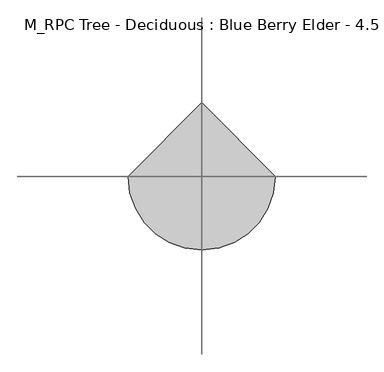
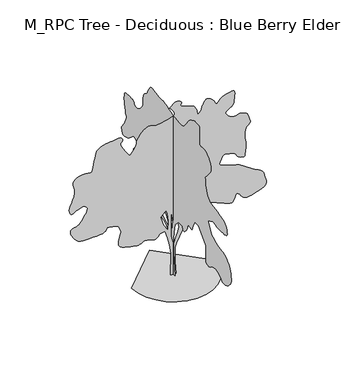
"""IFC4 building model written with IfcOpenShell, lengths in millimetres: geographic element geometry, M_RPC Tree - Deciduous : Blue Berry Elder - 4.5 Meters."""

from ifc_helpers import new_model, si_unit, origin, place, context, project, spatial, triangles, source, transform, mapped, element, save


def m_rpc_tree_deciduous_blue_berry_elder_4_5_meters_08da9c25(model_context):
    return source(origin(), model_context, "Body", "Tessellation", [
        triangles([(-0.0014684, 58.7037978, 0.0041346), (-0.0014684, -62.498052, 0.0041346), (-0.0014684, -15.3641626, 565.6129683), (-0.0014684, -1.8971866, 909.0182064), (-0.0014684, -22.0974929, 1104.2884094), (-0.0014684, -75.9650625, 1326.4911255), (-0.0014684, -224.1009287, 1474.6287403), (-0.0014684, -378.970291, 1474.6287403), (-0.0014684, -412.6378218, 1380.3586224), (-0.0014684, -479.9703761, 1387.0936764), (-0.0014684, -554.0404552, 1474.6287403), (-0.0014684, -601.1729708, 1568.8962421), (-0.0014684, -628.1080273, 1663.1638893), (-0.0014684, -702.1755266, 1636.2313763), (-0.0014684, -782.9756092, 1629.4963223), (-0.0014684, -857.0431812, 1797.8338669), (-0.0014684, -910.9107508, 1898.833952), (-0.0014684, -1059.0483656, 1892.1015141), (-0.0014684, -1173.5159426, 1797.8338669), (-0.0014684, -1382.2535648, 1575.6288254), (-0.0014684, -1388.9861481, 1353.4261093), (-0.0014684, -1386.9236286, 1327.021035), (-0.0014684, -1382.3910564, 1295.553479), (-0.0014684, -1377.8561588, 1261.3760593), (-0.0014684, -1375.7936394, 1226.8434288), (-0.0014684, -1378.6786377, 1194.3159811), (-0.0014684, -1388.9861481, 1166.1458982), (-0.0014684, -1409.1860779, 1144.6884144), (-0.0014684, -1434.4711624, 1129.1809307), (-0.0014684, -1458.931152, 1117.9109064), (-0.0014684, -1483.3911415, 1111.8258854), (-0.0014684, -1508.676226, 1111.8658539), (-0.0014684, -1535.6112099, 1118.9734142), (-0.0014684, -1565.0162464, 1134.0884073), (-0.0014684, -1597.723843, 1158.1559063), (-0.0014684, -1638.2812511, 1183.6959171), (-0.0014684, -1688.0263252, 1202.5209309), (-0.0014684, -1742.9539318, 1214.5159836), (-0.0014684, -1799.0589375, 1219.5610245), (-0.0014684, -1852.3364994, 1217.5409443), (-0.0014684, -1898.783955, 1208.3334394), (-0.0014684, -1934.3939907, 1191.8234734), (-0.0014684, -1963.8416119, 1167.0484594), (-0.0014684, -1995.1715309, 1136.2684341), (-0.0014684, -2029.446619, 1104.1908863), (-0.0014684, -2067.729166, 1075.5283916), (-0.0014684, -2111.0741947, 1054.9958513), (-0.0014684, -2160.5442856, 1047.2983561), (-0.0014684, -2217.1992577, 1057.1533504), (-0.0014684, -2275.1493542, 1083.4008762), (-0.0014684, -2327.094294, 1119.5408941), (-0.0014684, -2371.9694618, 1162.2784018), (-0.0014684, -2408.7193989, 1208.3134552), (-0.0014684, -2436.2819607, 1254.348436), (-0.0014684, -2453.5944214, 1297.0834728), (-0.0014684, -2459.6019035, 1333.2260342), (-0.0014684, -2455.754464, 1372.7236233), (-0.0014684, -2445.3120781, 1424.1161259), (-0.0014684, -2429.919413, 1481.9887562), (-0.0014684, -2411.2318909, 1540.9212055), (-0.0014684, -2390.8944695, 1595.4962173), (-0.0014684, -2370.5569027, 1640.2937737), (-0.0014684, -2351.8669098, 1669.8963272), (-0.0014684, -2330.1568977, 1694.4363991), (-0.0014684, -2300.1992786, 1725.2163517), (-0.0014684, -2262.8217636, 1758.5913494), (-0.0014684, -2218.8493023, 1790.903912), (-0.0014684, -2169.1042282, 1818.5039715), (-0.0014684, -2114.4116364, 1837.74146), (-0.0014684, -2055.5966217, 1844.9664551), (-0.0014684, -1994.4066067, 1849.8740044), (-0.0014684, -1932.1564819, 1863.6164795), (-0.0014684, -1869.0239983, 1884.7189705), (-0.0014684, -1805.1839996, 1911.7115089), (-0.0014684, -1740.8139462, 1943.1215103), (-0.0014684, -1676.0888271, 1977.4765354), (-0.0014684, -1611.1887188, 2013.3016743), (-0.0014684, -1469.786158, 2275.9068661), (-0.0014684, -1685.2562908, 2376.9094219), (-0.0014684, -1714.2713802, 2368.3093655), (-0.0014684, -1744.228854, 2360.0643745), (-0.0014684, -1776.0713871, 2352.5268986), (-0.0014684, -1810.7388931, 2346.049387), (-0.0014684, -1849.1765179, 2340.9844345), (-0.0014684, -1892.3265003, 2337.686816), (-0.0014684, -1941.1290447, 2336.5068008), (-0.0014684, -1996.881601, 2336.291843), (-0.0014684, -2057.3441895, 2336.4293346), (-0.0014684, -2118.1616982, 2338.0968201), (-0.0014684, -2174.9742188, 2342.4769306), (-0.0014684, -2223.421843, 2350.7393623), (-0.0014684, -2259.1517841, 2364.0693626), (-0.0014684, -2277.7993378, 2383.6418598), (-0.0014684, -2281.3742649, 2414.4819832), (-0.0014684, -2275.8767807, 2457.2194908), (-0.0014684, -2262.9592552, 2506.4269524), (-0.0014684, -2244.2692623, 2556.7020813), (-0.0014684, -2221.4593174, 2602.6271851), (-0.0014684, -2196.1742329, 2638.7770134), (-0.0014684, -2170.0641987, 2659.7021896), (-0.0014684, -2143.7191498, 2670.2021301), (-0.0014684, -2115.1367374, 2679.2771576), (-0.0014684, -2082.0791622, 2687.9772079), (-0.0014684, -2042.3065899, 2697.4022141), (-0.0014684, -1993.581657, 2708.6021118), (-0.0014684, -1933.6665642, 2722.6021294), (-0.0014684, -1860.3264187, 2740.5021996), (-0.0014684, -1781.7239491, 2758.3022758), (-0.0014684, -1708.0688519, 2773.1522415), (-0.0014684, -1640.1837513, 2787.8522163), (-0.0014684, -1578.8962132, 2805.302314), (-0.0014684, -1525.0287163, 2828.2773651), (-0.0014684, -1479.4062103, 2859.6021973), (-0.0014684, -1442.8536449, 2902.1272179), (-0.0014684, -1414.8411106, 2953.5272781), (-0.0014684, -1393.5411026, 3009.1773697), (-0.0014684, -1377.8361019, 3068.3775352), (-0.0014684, -1366.6061188, 3130.3775299), (-0.0014684, -1358.7336342, 3194.527684), (-0.0014684, -1353.1011292, 3260.0777527), (-0.0014684, -1348.5861431, 3326.3277786), (-0.0014684, -1398.7811897, 3378.2528069), (-0.0014684, -1447.1536732, 3430.0528427), (-0.0014684, -1491.8711472, 3481.6278923), (-0.0014684, -1531.1136646, 3532.8529633), (-0.0014684, -1563.0537209, 3583.577774), (-0.0014684, -1585.8662819, 3633.7529091), (-0.0014684, -1597.723843, 3683.2030884), (-0.0014684, -1593.7187096, 3737.8779488), (-0.0014684, -1572.2812099, 3799.8529449), (-0.0014684, -1536.5912373, 3863.2281464), (-0.0014684, -1489.8311554, 3922.153038), (-0.0014684, -1435.1786774, 3970.7032722), (-0.0014684, -1375.8135509, 4002.9783371), (-0.0014684, -1314.918576, 4013.128299), (-0.0014684, -1258.4585049, 4010.1031929), (-0.0014684, -1210.3634754, 4007.7533363), (-0.0014684, -1170.7484516, 4007.6533424), (-0.0014684, -1139.7309408, 4011.3281181), (-0.0014684, -1117.4309212, 4020.3031517), (-0.0014684, -1103.9633566, 4036.1033501), (-0.0014684, -1099.4483706, 4060.2783279), (-0.0014684, -1101.1558971, 4105.3531929), (-0.0014684, -1104.8659178, 4175.1532928), (-0.0014684, -1108.4583584, 4258.1534592), (-0.0014684, -1109.8133629, 4342.8035248), (-0.0014684, -1106.8083864, 4417.5536133), (-0.0014684, -1097.3283691, 4470.8785561), (-0.0014684, -1079.2483681, 4491.2034782), (-0.0014684, -1052.7858118, 4492.578685), (-0.0014684, -1020.9033102, 4495.6035004), (-0.0014684, -985.6082989, 4498.6286064), (-0.0014684, -948.8982576, 4500.0035225), (-0.0014684, -912.7757532, 4498.07864), (-0.0014684, -879.2456778, 4491.2034782), (-0.0014684, -850.3106707, 4477.7537178), (-0.0014684, -822.8281912, 4461.7535316), (-0.0014684, -792.8706448, 4447.2035477), (-0.0014684, -761.2631264, 4432.1535942), (-0.0014684, -728.8330564, 4414.7534935), (-0.0014684, -696.4030592, 4393.1286507), (-0.0014684, -664.7980116, 4365.3786003), (-0.0014684, -634.8405378, 4329.6034584), (-0.0014684, -604.8054889, 4286.4284775), (-0.0014684, -572.6504748, 4239.8534134), (-0.0014684, -538.7279451, 4193.0283646), (-0.0014684, -503.3903855, 4149.1534264), (-0.0014684, -466.9953687, 4111.403405), (-0.0014684, -429.8928369, 4082.9533974), (-0.0014684, -392.4378193, 4067.0032082), (-0.0014684, -354.0977903, 4061.0282822), (-0.0014684, -314.1102602, 4059.6533661), (-0.0014684, -272.4727218, 4061.703241), (-0.0014684, -229.185175, 4065.9782707), (-0.0014684, -184.2498909, 4071.3282349), (-0.0014684, -137.6653616, 4076.5532066), (-0.0014684, -89.4320684, 4080.4782578), (-0.0014684, -32.5020268, 4087.803392), (-0.0014684, 35.3820291, 4102.1033913), (-0.0014684, 107.0353362, 4120.403437), (-0.0014684, 175.2726409, 4139.7534187), (-0.0014684, 232.909439, 4157.2282242), (-0.0014684, 272.7602224, 4169.8783241), (-0.0014684, 287.6402371, 4174.7283188), (-0.0014684, 295.8277279, 4177.2784538), (-0.0014684, 318.5002539, 4183.6033585), (-0.0014684, 352.8352947, 4191.7034454), (-0.0014684, 396.002827, 4199.553257), (-0.0014684, 445.1803485, 4205.1534966), (-0.0014684, 497.5354013, 4206.5284126), (-0.0014684, 550.2454471, 4201.678418), (-0.0014684, 608.3329988, 4200.728476), (-0.0014684, 675.2555128, 4211.4534027), (-0.0014684, 745.8280947, 4228.1782539), (-0.0014684, 814.8706827, 4245.2533745), (-0.0014684, 877.2006718, 4257.0285278), (-0.0014684, 927.6307331, 4257.8534775), (-0.0014684, 960.9857466, 4242.0782776), (-0.0014684, 983.9932812, 4214.9534798), (-0.0014684, 1006.5283155, 4185.8032242), (-0.0014684, 1028.123291, 4155.1533508), (-0.0014684, 1048.3033092, 4123.4282524), (-0.0014684, 1066.5983408, 4091.1031906), (-0.0014684, 1082.5408997, 4058.6781349), (-0.0014684, 1095.6533987, 4026.6033485), (-0.0014684, 1111.3183582, 3999.2282753), (-0.0014684, 1133.5808802, 3978.353096), (-0.0014684, 1159.9634268, 3960.5283119), (-0.0014684, 1187.9984161, 3942.3532585), (-0.0014684, 1215.2059851, 3920.4031448), (-0.0014684, 1239.1159355, 3891.2531799), (-0.0014684, 1257.255962, 3851.5279884), (-0.0014684, 1268.2685165, 3817.1530518), (-0.0014684, 1273.6285091, 3800.8031776), (-0.0014684, 1275.1009483, 3794.1030052), (-0.0014684, 1274.4534588, 3788.7030441), (-0.0014684, 1273.451049, 3776.252932), (-0.0014684, 1273.8635239, 3748.3528908), (-0.0014684, 1277.4560371, 3696.6528488), (-0.0014684, 1283.7985279, 3637.6029648), (-0.0014684, 1291.9060272, 3591.1778915), (-0.0014684, 1302.7210648, 3554.2528198), (-0.0014684, 1317.1884956, 3523.8279327), (-0.0014684, 1336.2511402, 3496.8278366), (-0.0014684, 1360.8486214, 3470.1527206), (-0.0014684, 1391.9260849, 3440.8027679), (-0.0014684, 1427.2211689, 3411.5778076), (-0.0014684, 1463.2262386, 3387.677813), (-0.0014684, 1498.9912067, 3369.4027657), (-0.0014684, 1533.5812466, 3357.1526413), (-0.0014684, 1566.0512123, 3351.2777092), (-0.0014684, 1595.4587196, 3352.1026588), (-0.0014684, 1620.8612389, 3360.002758), (-0.0014684, 1639.7087803, 3375.502684), (-0.0014684, 1652.8988182, 3396.6528465), (-0.0014684, 1664.6787678, 3420.0528717), (-0.0014684, 1679.2838356, 3442.2776779), (-0.0014684, 1700.9563499, 3459.9027649), (-0.0014684, 1733.936459, 3469.5277588), (-0.0014684, 1782.4638748, 3467.7278687), (-0.0014684, 1840.5514629, 3464.2277916), (-0.0014684, 1897.5815575, 3466.9779144), (-0.0014684, 1950.8390625, 3469.852739), (-0.0014684, 1997.6215267, 3466.7026405), (-0.0014684, 2035.2141449, 3451.4277008), (-0.0014684, 2060.9117043, 3417.9027122), (-0.0014684, 2072.001725, 3360.002758), (-0.0014684, 2074.396637, 3302.252504), (-0.0014684, 2075.4967152, 3266.6526421), (-0.0014684, 2074.8291687, 3243.2026199), (-0.0014684, 2071.9241135, 3221.8774681), (-0.0014684, 2066.3091946, 3192.6275093), (-0.0014684, 2057.5140919, 3145.5024788), (-0.0014684, 2045.0690666, 3070.4524086), (-0.0014684, 2028.7941879, 2993.7774376), (-0.0014684, 2011.3440903, 2941.8274109), (-0.0014684, 1996.4816254, 2904.7273499), (-0.0014684, 1987.9815628, 2872.5772774), (-0.0014684, 1989.6115505, 2835.4772163), (-0.0014684, 2005.1390911, 2783.5271896), (-0.0014684, 2038.3341579, 2706.8522186), (-0.0014684, 2081.1516026, 2626.4521843), (-0.0014684, 2121.1391327, 2566.6770538), (-0.0014684, 2155.4742462, 2522.5771294), (-0.0014684, 2181.326738, 2489.1794586), (-0.0014684, 2195.8742512, 2461.5570168), (-0.0014684, 2196.286726, 2434.7619953), (-0.0014684, 2179.7367187, 2403.841935), (-0.0014684, 2160.4392048, 2371.8244125), (-0.0014684, 2149.859182, 2345.5768867), (-0.0014684, 2141.0441677, 2325.9269234), (-0.0014684, 2127.0467663, 2313.6968559), (-0.0014684, 2100.919146, 2309.7117794), (-0.0014684, 2055.7091148, 2314.7967888), (-0.0014684, 1984.4665157, 2329.7743629), (-0.0014684, 1906.7289642, 2358.6118469), (-0.0014684, 1844.06651, 2399.6994553), (-0.0014684, 1792.5939251, 2445.4995667), (-0.0014684, 1748.4239468, 2488.4719437), (-0.0014684, 1707.671347, 2521.0769302), (-0.0014684, 1666.4437763, 2535.7769051), (-0.0014684, 1620.8612389, 2525.0519783), (-0.0014684, 1576.9086891, 2499.6619583), (-0.0014684, 1542.1411892, 2475.3396057), (-0.0014684, 1515.031216, 2451.8994667), (-0.0014684, 1494.0461597, 2429.166988), (-0.0014684, 1477.653701, 2406.9644188), (-0.0014684, 1464.3237007, 2385.1144444), (-0.0014684, 1452.526165, 2363.44193), (-0.0014684, 1471.2737125, 2344.7718487), (-0.0014684, 1489.9612347, 2326.634293), (-0.0014684, 1508.5336475, 2309.5543762), (-0.0014684, 1526.9262749, 2294.0668041), (-0.0014684, 1545.0862129, 2280.6968353), (-0.0014684, 1562.9512562, 2269.9793209), (-0.0014684, 1580.4612339, 2262.4393742), (-0.0014684, 1599.1313152, 2259.024321), (-0.0014684, 1619.331245, 2258.1993713), (-0.0014684, 1639.2963055, 2256.7868122), (-0.0014684, 1657.2588718, 2251.6042797), (-0.0014684, 1671.4513195, 2239.4717354), (-0.0014684, 1680.1087852, 2217.2092861), (-0.0014684, 1681.4637897, 2181.6392189), (-0.0014684, 1676.9863014, 2141.9842266), (-0.0014684, 1669.5664055, 2107.6292015), (-0.0014684, 1659.5537899, 2075.6315907), (-0.0014684, 1647.3038109, 2043.0441902), (-0.0014684, 1633.1712433, 2006.9215405), (-0.0014684, 1617.5037403, 1964.3241405), (-0.0014684, 1600.6613091, 1912.3015892), (-0.0014684, 1583.268766, 1853.7415009), (-0.0014684, 1567.0537674, 1795.0639778), (-0.0014684, 1554.0188072, 1738.6264343), (-0.0014684, 1546.1662342, 1686.7788723), (-0.0014684, 1545.4986877, 1641.8837929), (-0.0014684, 1554.0188072, 1606.2938141), (-0.0014684, 1573.728796, 1582.3637341), (-0.0014684, 1599.1112583, 1566.4212479), (-0.0014684, 1623.4337563, 1552.9562267), (-0.0014684, 1646.8737499, 1541.5487835), (-0.0014684, 1669.606374, 1531.7937103), (-0.0014684, 1691.8087978, 1523.2737362), (-0.0014684, 1713.6589176, 1515.5787117), (-0.0014684, 1735.331432, 1508.2936913), (-0.0014684, 1758.2389, 1518.0512352), (-0.0014684, 1780.0888744, 1525.7462597), (-0.0014684, 1799.8189201, 1529.318716), (-0.0014684, 1816.3664566, 1526.7087009), (-0.0014684, 1828.676461, 1515.8536949), (-0.0014684, 1835.6840275, 1494.6911785), (-0.0014684, 1836.331517, 1461.1611031), (-0.0014684, 1830.501495, 1425.4711304), (-0.0014684, 1819.3715057, 1398.2636341), (-0.0014684, 1803.8239082, 1378.1211136), (-0.0014684, 1784.7414974, 1363.6336258), (-0.0014684, 1763.0089577, 1353.3861408), (-0.0014684, 1739.5114094, 1345.9660995), (-0.0014684, 1715.128886, 1339.9586174), (-0.0014684, 1703.5663651, 1332.6360992), (-0.0014684, 1691.8864094, 1324.6660915), (-0.0014684, 1679.9712936, 1315.4011047), (-0.0014684, 1667.701403, 1304.1910332), (-0.0014684, 1654.9613377, 1290.3910034), (-0.0014684, 1641.6313374, 1273.3510551), (-0.0014684, 1627.5962929, 1252.4235535), (-0.0014684, 1608.2588104, 1230.1234612), (-0.0014684, 1580.0887276, 1209.2360006), (-0.0014684, 1544.5563034, 1189.5259392), (-0.0014684, 1503.1336864, 1170.7584074), (-0.0014684, 1457.2962227, 1152.6983906), (-0.0014684, 1408.5135899, 1135.1084032), (-0.0014684, 1358.2585178, 1117.7559013), (-0.0014684, 1196.6559546, 1212.0234758), (-0.0014684, 1035.0533186, 1090.8208448), (-0.0014684, 1013.4382862, 1088.0133854), (-0.0014684, 992.0007866, 1085.6783535), (-0.0014684, 970.9182798, 1084.2833805), (-0.0014684, 950.3632845, 1084.3033648), (-0.0014684, 930.5182749, 1086.2083357), (-0.0014684, 911.5532261, 1090.4683954), (-0.0014684, 893.6506851, 1097.5558989), (-0.0014684, 877.0431959, 1106.938393), (-0.0014684, 861.3756929, 1117.3809242), (-0.0014684, 845.9456755, 1128.295883), (-0.0014684, 830.0456285, 1139.0934071), (-0.0014684, 812.9656391, 1149.1834162), (-0.0014684, 794.0031338, 1157.9784462), (-0.0014684, 772.4481268, 1164.8884169), (-0.0014684, 748.1855816, 1170.2684664), (-0.0014684, 721.8005642, 1174.9409283), (-0.0014684, 693.6505383, 1179.0234552), (-0.0014684, 664.0855551, 1182.6359528), (-0.0014684, 633.4605349, 1185.8934574), (-0.0014684, 602.1304705, 1188.9184181), (-0.0014684, 570.4454495, 1191.8234734), (-0.0014684, 361.7077909, 1131.2209225), (-0.0014684, 186.6391528, 1003.2857809), (-0.0014684, 92.3710696, 848.418199), (-0.0014684, 45.2367873, 552.1454401), (-0.0013758, 65.4370532, 1097.5558989), (-0.0013758, 166.4388778, 1313.0261044), (-0.0013758, 4.8361539, 1380.3586224), (-0.0013882, 307.8402577, 1171.6234709), (-0.0013882, 469.4428937, 1279.3585373), (-0.0013882, 597.3779626, 1286.0909752), (-0.0013882, 705.1130653, 1346.6910553), (-0.0013882, 699.3030275, 1349.8135391), (-0.0013882, 693.2555769, 1354.3485821), (-0.0013882, 686.7405676, 1361.7110687), (-0.0013882, 679.5155725, 1373.3110874), (-0.0013882, 671.3480478, 1390.5686096), (-0.0013882, 662.0055222, 1414.8911076), (-0.0013882, 651.2454958, 1447.6936111), (-0.0013882, 642.6479828, 1480.1036968), (-0.0013882, 639.3505096, 1503.3287327), (-0.0013882, 640.4680286, 1518.8962418), (-0.0013882, 645.1205063, 1528.3386887), (-0.0013882, 652.425511, 1533.1862125), (-0.0013882, 661.4930534, 1534.9737488), (-0.0013882, 671.4480417, 1535.2286751), (-0.0013882, 678.1805523, 1616.0288303), (-0.0013882, 597.3779626, 1669.8963272), (-0.0013882, 422.3103418, 1521.7611832), (-0.0013882, 301.1077472, 1380.3586224), (-0.0013882, 220.3061749, 1265.8910454), (-0.0013882, 139.504866, 1084.0883343), (66.6360534, 0.0002629, 0.0), (-68.0330566, 0.0002629, 0.0), (-61.2998012, 0.0002272, 552.142933), (-94.9670776, 0.0002139, 794.5456152), (-142.1008648, 0.0002005, 996.5483288), (-202.7016535, 0.0001916, 1178.3509672), (-323.9027584, 0.0001916, 1164.8859461), (-344.1627863, 0.0001916, 1136.3209019), (-364.7752999, 0.000196, 1109.5258804), (-386.0952922, 0.000196, 1086.2633469), (-408.4753215, 0.000196, 1068.3008532), (-432.2678372, 0.0002005, 1057.4058786), (-457.8253615, 0.0002005, 1055.3433592), (-485.5053944, 0.000196, 1063.8833176), (-514.9529065, 0.000196, 1076.7408903), (-545.4604194, 0.000196, 1086.7733448), (-576.8504728, 0.000196, 1094.448385), (-608.9454978, 0.000196, 1100.2409094), (-641.5730484, 0.000196, 1104.6184038), (-674.5530121, 0.000196, 1108.0533686), (-707.7105812, 0.000196, 1111.0183765), (-735.2131176, 0.000196, 1095.3133759), (-763.2456362, 0.000196, 1080.6083868), (-792.3406626, 0.000196, 1067.9083626), (-823.0231647, 0.000196, 1058.210844), (-855.8256683, 0.0002005, 1052.5183136), (-891.280699, 0.0002005, 1051.8308556), (-929.9132246, 0.0002005, 1057.1508797), (-979.8558157, 0.000196, 1066.7883728), (-1044.1658438, 0.000196, 1079.0183676), (-1115.7808765, 0.000196, 1094.7833937), (-1187.630924, 0.000196, 1115.0233646), (-1252.6485397, 0.0001916, 1140.6808828), (-1303.7660591, 0.0001916, 1172.6984053), (-1333.9185791, 0.0001871, 1212.0184616), (-1343.6560661, 0.0001871, 1258.8785374), (-1340.9085594, 0.0001827, 1310.6835148), (-1329.6785763, 0.0001782, 1364.141153), (-1313.9735756, 0.0001782, 1415.9461304), (-1297.7985455, 0.0001738, 1462.8062061), (-1285.1560032, 0.0001738, 1501.4186749), (-1280.0510822, 0.0001693, 1528.4911503), (-1282.3885849, 0.0001693, 1551.6362492), (-1288.8460396, 0.0001693, 1579.2562202), (-1298.6035835, 0.0001648, 1609.2337509), (-1310.8335056, 0.0001648, 1639.4462963), (-1324.7136177, 0.0001604, 1667.7737823), (-1339.4160633, 0.0001604, 1692.0964256), (-1354.121125, 0.0001604, 1710.2938614), (-1373.4561367, 0.0001604, 1723.3488785), (-1401.6286903, 0.0001559, 1733.9289013), (-1437.1586437, 0.0001559, 1742.4488754), (-1478.5811153, 0.0001559, 1749.3189503), (-1524.4187244, 0.0001559, 1754.9539261), (-1573.2012119, 0.0001559, 1759.7639523), (-1623.456284, 0.0001559, 1764.1613583), (-1631.2713593, 0.0001559, 1738.3664211), (-1642.6763317, 0.0001604, 1713.631303), (-1661.2663307, 0.0001604, 1691.0164043), (-1690.6363403, 0.0001604, 1671.5813988), (-1734.3739323, 0.0001604, 1656.386396), (-1796.0739452, 0.0001648, 1646.4938313), (-1879.3290379, 0.0001648, 1642.9588726), (-1971.5741341, 0.0001648, 1640.6613384), (-2057.4616241, 0.0001648, 1636.1262955), (-2136.396777, 0.0001648, 1632.8888477), (-2207.7943085, 0.0001648, 1634.478867), (-2271.0667545, 0.0001648, 1644.4313118), (-2325.619384, 0.0001604, 1666.2812862), (-2370.8693836, 0.0001604, 1703.5614235), (-2411.8019142, 0.0001559, 1752.5588688), (-2450.9643494, 0.0001559, 1805.3264328), (-2484.1219185, 0.0001515, 1859.0389973), (-2507.0269157, 0.000147, 1910.8640316), (-2515.4519829, 0.0001426, 1957.9790337), (-2505.1520302, 0.0001426, 1997.554089), (-2471.8720848, 0.0001426, 2026.7640793), (-2428.4668854, 0.0001381, 2045.1190636), (-2390.1269291, 0.0001381, 2056.5266521), (-2356.1468811, 0.0001381, 2064.7515862), (-2325.816901, 0.0001381, 2073.5666004), (-2298.4317993, 0.0001381, 2086.7391975), (-2273.2843517, 0.0001337, 2108.0367348), (-2249.6667526, 0.0001337, 2141.2342724), (-2221.7142437, 0.0001292, 2184.9518074), (-2187.6342018, 0.0001292, 2233.7342949), (-2152.8467903, 0.0001247, 2285.2267914), (-2122.7717365, 0.0001203, 2337.0718826), (-2102.826733, 0.0001203, 2386.9169506), (-2098.4291817, 0.0001158, 2432.401965), (-2114.9992458, 0.0001158, 2471.1718369), (-2145.426749, 0.0001114, 2498.537027), (-2178.6816959, 0.0001114, 2512.8271431), (-2214.2917316, 0.0001114, 2516.2269356), (-2251.7868267, 0.0001114, 2510.9019699), (-2290.6968063, 0.0001114, 2499.0494957), (-2330.5468449, 0.0001114, 2482.831881), (-2370.8693836, 0.0001158, 2464.439399), (-2399.569376, 0.0001158, 2448.8118645), (-2427.3294548, 0.0001158, 2434.6593853), (-2453.2020035, 0.0001158, 2423.4494591), (-2476.2471085, 0.0001158, 2416.6569958), (-2495.5270363, 0.0001158, 2415.7544346), (-2510.1020187, 0.0001158, 2422.2118893), (-2519.0020569, 0.0001158, 2437.5044151), (-2525.7269371, 0.0001158, 2456.4494797), (-2533.1520653, 0.0001158, 2474.4518692), (-2539.5019684, 0.0001114, 2493.8669632), (-2543.0270439, 0.0001114, 2517.0518852), (-2541.977108, 0.0001114, 2546.3521317), (-2534.5519798, 0.0001069, 2584.15215), (-2519.0020569, 0.0001025, 2632.7770889), (-2498.1969315, 0.0001025, 2684.6521202), (-2477.0345604, 9.8e-05, 2732.0771324), (-2456.8145737, 9.8e-05, 2777.1272896), (-2438.8319504, 9.36e-05, 2821.9271713), (-2424.3844311, 8.91e-05, 2868.6522263), (-2414.7643787, 8.91e-05, 2919.3523293), (-2411.2693886, 8.47e-05, 2976.1773491), (-2415.2169674, 8.02e-05, 3030.6775108), (-2424.696912, 8.02e-05, 3074.9274261), (-2436.1819668, 7.57e-05, 3111.8774963), (-2446.1344116, 7.57e-05, 3144.4525429), (-2451.0245201, 7.13e-05, 3175.6276749), (-2447.311956, 7.13e-05, 3208.3274231), (-2431.4719345, 6.68e-05, 3245.527478), (-2401.6519524, 6.68e-05, 3281.1526291), (-2361.1144558, 6.24e-05, 3307.9527374), (-2313.9793968, 6.24e-05, 3326.977739), (-2264.3718143, 6.24e-05, 3339.2775696), (-2216.4142765, 6.24e-05, 3345.9277451), (-2174.2267353, 6.24e-05, 3348.0026184), (-2141.9342297, 6.24e-05, 3346.5277084), (-2114.2341763, 6.24e-05, 3341.002755), (-2084.4141941, 6.24e-05, 3332.902668), (-2054.4766319, 6.24e-05, 3326.2027863), (-2026.4241291, 6.24e-05, 3324.9275734), (-2002.2565636, 6.24e-05, 3333.0776573), (-1983.9815163, 6.24e-05, 3354.6527939), (-1973.5965397, 5.79e-05, 3393.652739), (-1964.8216393, 5.35e-05, 3450.0277863), (-1951.2165104, 5.35e-05, 3517.3777451), (-1934.5515392, 4.9e-05, 3590.1279556), (-1916.5889729, 4.46e-05, 3662.7528831), (-1899.0965813, 4.01e-05, 3729.7278648), (-1883.8440239, 3.56e-05, 3785.5279472), (-1872.5939838, 3.12e-05, 3824.6031784), (-1852.5114887, 3.12e-05, 3852.8781967), (-1813.3489082, 3.12e-05, 3879.4030312), (-1760.7564789, 2.67e-05, 3903.2280304), (-1700.3914135, 2.67e-05, 3923.3782539), (-1637.906274, 2.67e-05, 3938.9531754), (-1578.9537678, 2.67e-05, 3948.9781448), (-1529.1887821, 2.67e-05, 3952.5282188), (-1482.7811497, 2.67e-05, 3955.978299), (-1432.4861092, 2.67e-05, 3963.6781197), (-1381.8386192, 2.67e-05, 3971.6032173), (-1334.3710224, 2.23e-05, 3975.7782532), (-1293.6160973, 2.67e-05, 3972.1531837), (-1263.1109825, 2.67e-05, 3956.7782501), (-1246.3835152, 2.67e-05, 3925.6031181), (-1245.9735111, 3.12e-05, 3891.2531799), (-1257.1035004, 3.12e-05, 3865.2780212), (-1272.3560577, 3.12e-05, 3842.0279869), (-1284.3134674, 3.56e-05, 3815.8281326), (-1285.5485664, 3.56e-05, 3781.0029327), (-1268.6459644, 4.01e-05, 3731.9530197), (-1226.1859108, 4.46e-05, 3663.0028679), (-1175.7534513, 4.9e-05, 3589.303006), (-1137.6884056, 4.9e-05, 3530.2028343), (-1108.6933731, 5.35e-05, 3486.3028976), (-1085.4708807, 5.35e-05, 3458.2028687), (-1064.7208391, 5.79e-05, 3446.4527138), (-1043.1458479, 5.35e-05, 3451.6776855), (-1017.4482885, 5.35e-05, 3474.4527489), (-990.2407923, 5.35e-05, 3507.3527756), (-966.3282984, 4.9e-05, 3542.2529709), (-945.7157484, 4.9e-05, 3578.7027809), (-928.403215, 4.46e-05, 3616.2028175), (-914.3857567, 4.46e-05, 3654.2778191), (-903.6682423, 4.01e-05, 3692.477813), (-896.2457302, 4.01e-05, 3730.3281189), (-882.6607309, 3.56e-05, 3773.9530724), (-855.1781788, 3.12e-05, 3826.1530838), (-816.3881773, 3.12e-05, 3881.5531906), (-768.880612, 2.67e-05, 3934.7281425), (-715.2480572, 2.23e-05, 3980.2282722), (-658.0830145, 2.23e-05, 4012.6533279), (-599.9754785, 2.23e-05, 4026.6033485), (-552.8204352, 2.23e-05, 4024.7781693), (-521.215424, 2.23e-05, 4016.1031174), (-496.7928958, 2.23e-05, 4004.503244), (-471.1953667, 2.23e-05, 3993.8533127), (-436.0553604, 2.23e-05, 3988.0280869), (-383.0128132, 2.23e-05, 3990.9032021), (-303.7027378, 2.23e-05, 4006.4031281), (-214.7551692, 2.23e-05, 4026.5783501), (-138.763614, 2.23e-05, 4042.5282486), (-76.3173075, 1.78e-05, 4056.5782631), (-28.0055217, 1.78e-05, 4071.1032486), (5.5830293, 1.78e-05, 4088.4533524), (23.8594698, 1.78e-05, 4110.9784309), (26.2347699, 1.34e-05, 4141.0533394), (18.3040142, 1.34e-05, 4173.7283798), (6.4862053, 8.9e-06, 4202.8533463), (-8.5707069, 8.9e-06, 4229.0534912), (-26.219021, 8.9e-06, 4252.8784904), (-45.810535, 4.5e-06, 4274.9533058), (-66.6978047, 4.5e-06, 4295.8284851), (-88.2330682, 4.5e-06, 4316.1284088), (-60.8870493, 4.5e-06, 4341.9035797), (-33.9532782, 0.0, 4366.5035316), (-7.8441564, 0.0, 4388.753627), (17.0283131, 0.0, 4407.4536484), (40.2517809, 0.0, 4421.4536659), (61.4140475, -4.5e-06, 4429.5534622), (80.1028141, -4.5e-06, 4430.6036888), (99.5373291, -4.5e-06, 4426.853627), (121.7990971, 0.0, 4421.2286797), (144.7671174, 0.0, 4413.4535728), (166.3221335, 0.0, 4403.3536079), (184.343399, 0.0, 4390.653511), (196.7109036, 0.0, 4375.1285866), (201.3046639, 0.0, 4356.5285591), (197.1231604, 4.5e-06, 4339.6534264), (187.641399, 4.5e-06, 4327.8285667), (177.4531401, 4.5e-06, 4318.7285408), (171.1516352, 4.5e-06, 4309.9784935), (173.3306447, 4.5e-06, 4299.2035698), (188.5838924, 4.5e-06, 4284.1033287), (221.5051751, 8.9e-06, 4262.2784981), (265.7927153, 8.9e-06, 4240.0534012), (311.140238, 8.9e-06, 4223.8285194), (356.135275, 8.9e-06, 4211.3784073), (399.3628326, 8.9e-06, 4200.4784912), (439.4103518, 1.34e-05, 4188.8533287), (474.8628754, 1.34e-05, 4174.2783463), (504.3103875, 1.34e-05, 4154.528389), (527.7304333, 1.34e-05, 4129.0781982), (546.555447, 1.78e-05, 4099.4032654), (561.5529327, 1.78e-05, 4066.203257), (573.4879601, 2.23e-05, 4030.1531319), (583.1279603, 2.23e-05, 3991.9781364), (591.2354596, 2.67e-05, 3952.4032265), (598.577962, 2.67e-05, 3912.1280685), (692.8455729, 2.23e-05, 3999.6532494), (692.2180676, 2.23e-05, 4003.2033234), (691.118062, 2.23e-05, 4013.1033005), (690.7255714, 2.23e-05, 4028.2782463), (692.2180676, 2.23e-05, 4047.7282219), (696.7730221, 1.78e-05, 4070.3282959), (705.5680521, 1.78e-05, 4095.0782387), (719.7805567, 1.78e-05, 4120.8534096), (736.0730942, 1.34e-05, 4147.7032242), (751.1906307, 1.34e-05, 4174.7783157), (766.4231312, 8.9e-06, 4199.8282402), (783.0706615, 8.9e-06, 4220.678421), (802.4256575, 8.9e-06, 4235.0284172), (825.7856415, 8.9e-06, 4240.6533646), (854.4482088, 8.9e-06, 4235.3283989), (884.2282225, 8.9e-06, 4222.4283142), (910.4757483, 8.9e-06, 4207.0283821), (933.7782503, 1.34e-05, 4189.5782845), (954.7232655, 1.34e-05, 4170.4782875), (973.9032721, 1.34e-05, 4150.1283669), (991.9032635, 1.34e-05, 4128.9782043), (1009.3183342, 1.78e-05, 4107.4033585), (1013.7732948, 1.78e-05, 4086.0282097), (1018.9957958, 1.78e-05, 4066.2282555), (1025.7482906, 1.78e-05, 4049.6281059), (1034.7983196, 2.23e-05, 4037.7782478), (1046.910807, 2.23e-05, 4032.3032913), (1062.8508224, 2.23e-05, 4034.7781403), (1083.3858335, 2.23e-05, 4046.8032784), (1105.9033545, 1.78e-05, 4067.7281639), (1128.3008972, 1.78e-05, 4093.828315), (1152.1133972, 1.78e-05, 4122.0533363), (1178.8709209, 1.34e-05, 4149.3534142), (1210.1034622, 1.34e-05, 4172.628447), (1247.3434856, 1.34e-05, 4188.8533287), (1292.120985, 1.34e-05, 4194.9282486), (1340.4335884, 8.9e-06, 4200.0782249), (1385.9186028, 8.9e-06, 4211.3534088), (1426.5736794, 8.9e-06, 4222.5033096), (1460.3986496, 8.9e-06, 4227.2783089), (1485.388694, 8.9e-06, 4219.4784943), (1499.543644, 1.34e-05, 4192.8033783), (1500.85868, 1.34e-05, 4141.0533394), (1496.0287422, 1.78e-05, 4077.628141), (1491.9061741, 2.23e-05, 4020.1781593), (1486.7236416, 2.67e-05, 3968.9780869), (1478.7161362, 2.67e-05, 3924.2532005), (1466.111237, 3.12e-05, 3886.2531944), (1447.1485863, 3.12e-05, 3855.2030548), (1420.05867, 3.12e-05, 3831.3280586), (1386.1536175, 3.56e-05, 3811.7280922), (1350.8386219, 3.56e-05, 3792.5031029), (1318.4660339, 3.56e-05, 3772.3278809), (1293.3985233, 3.56e-05, 3749.9030869), (1279.9910568, 4.01e-05, 3723.9529266), (1282.6010719, 4.01e-05, 3693.1530624), (1305.5884769, 4.46e-05, 3656.2529892), (1339.7660419, 4.46e-05, 3620.9528183), (1372.8836426, 4.9e-05, 3594.8529579), (1404.7061188, 4.9e-05, 3576.4029213), (1434.9961304, 4.9e-05, 3564.0778015), (1463.5211334, 4.9e-05, 3556.3279839), (1490.0411716, 4.9e-05, 3551.6529785), (1514.3261719, 4.9e-05, 3548.5278786), (1534.9186649, 4.9e-05, 3550.0027885), (1552.0962502, 4.9e-05, 3557.8278923), (1568.2112549, 4.9e-05, 3568.4778236), (1585.6263256, 4.9e-05, 3578.4527962), (1606.6888481, 4.9e-05, 3584.152739), (1633.7613235, 4.9e-05, 3582.1028641), (1669.1938992, 4.9e-05, 3568.7278084), (1706.7689312, 4.9e-05, 3552.8279068), (1738.9239452, 4.9e-05, 3542.9279297), (1766.0138615, 4.9e-05, 3535.1528229), (1788.3938908, 4.9e-05, 3525.6028244), (1806.4140118, 5.35e-05, 3510.4278786), (1820.4314701, 5.35e-05, 3485.6776451), (1830.7965351, 5.79e-05, 3447.5276482), (1843.1639488, 5.79e-05, 3405.1526184), (1859.6539307, 6.24e-05, 3369.1527809), (1875.3189629, 6.24e-05, 3337.6276703), (1885.2139984, 6.24e-05, 3308.7026917), (1884.3890488, 6.68e-05, 3280.4526718), (1867.8990669, 6.68e-05, 3251.0527222), (1830.7965351, 7.13e-05, 3218.5776695), (1790.6914249, 7.13e-05, 3174.2274696), (1766.368927, 7.57e-05, 3114.4526299), (1754.6488575, 8.02e-05, 3045.2524933), (1752.3514687, 8.47e-05, 2972.6522736), (1756.2964314, 8.91e-05, 2902.6271873), (1763.3064686, 9.36e-05, 2841.2021576), (1770.196455, 9.36e-05, 2794.3771088), (1774.2014431, 9.8e-05, 2756.2771088), (1775.0263927, 9.8e-05, 2717.1021744), (1773.198888, 0.0001025, 2677.0520027), (1769.2539253, 0.0001025, 2636.3021645), (1763.7189434, 0.0001069, 2595.0270676), (1757.121381, 0.0001069, 2553.3769936), (1749.9963799, 0.0001114, 2511.5769287), (1751.0764011, 0.0001114, 2490.1945129), (1749.9764683, 0.0001158, 2470.407058), (1744.5189526, 0.0001158, 2453.7993507), (1732.5238998, 0.0001158, 2441.9619919), (1711.8138268, 0.0001158, 2436.4844193), (1680.2063084, 0.0001158, 2438.9569427), (1635.5263321, 0.0001158, 2450.971907), (1592.8687614, 0.0001158, 2472.329615), (1564.6988239, 0.0001114, 2499.8145653), (1544.8911667, 0.0001114, 2530.4769379), (1527.3211636, 0.0001069, 2561.3770866), (1505.8637524, 0.0001069, 2589.5771095), (1474.3961964, 0.0001069, 2612.1021881), (1426.7911079, 0.0001069, 2626.0522087), (1373.8061153, 0.0001025, 2635.8521919), (1329.4210339, 0.0001025, 2646.0271523), (1292.338559, 0.0001025, 2653.6019806), (1261.2609501, 0.0001025, 2655.6521461), (1234.8984604, 0.0001025, 2649.2022491), (1211.9484804, 0.0001025, 2631.3521759), (1191.1209726, 0.0001069, 2599.1021095), (1170.9584679, 0.0001069, 2559.6521919), (1152.6834206, 0.0001114, 2522.5521309), (1139.0008982, 0.0001114, 2488.5071159), (1132.6209097, 0.0001158, 2458.2345451), (1136.2509207, 0.0001158, 2432.4394627), (1152.6034109, 0.0001158, 2411.8269127), (1184.3859186, 0.0001203, 2397.1044102), (1219.3110397, 0.0001203, 2386.6219105), (1246.1060612, 0.0001203, 2377.5519699), (1269.016, 0.0001203, 2368.8369495), (1292.2785336, 0.0001203, 2359.4119434), (1320.1359901, 0.0001203, 2348.2243996), (1356.8260471, 0.0001203, 2334.2067959), (1406.5911781, 0.0001247, 2316.3044003), (1459.7311031, 0.0001247, 2299.7343361), (1505.2162628, 0.0001247, 2288.4668552), (1545.2837299, 0.0001247, 2279.5543179), (1582.1713039, 0.0001247, 2270.0518456), (1618.1137321, 0.0001247, 2257.01674), (1655.3537556, 0.0001292, 2237.5042683), (1696.128883, 0.0001292, 2208.5692612), (1938.5315289, 0.0001381, 2040.2315712), (1981.0741356, 0.0001426, 2013.7116783), (2030.6815727, 0.0001426, 1989.6615475), (2082.8791134, 0.0001426, 1964.7890831), (2133.1942108, 0.000147, 1935.7940506), (2177.1467606, 0.000147, 1899.3789768), (2210.2642159, 0.0001515, 1852.246534), (2228.0692337, 0.0001559, 1791.0938713), (2241.2617424, 0.0001604, 1726.50886), (2258.5768192, 0.0001604, 1670.1688396), (2272.5942776, 0.0001648, 1620.4237656), (2275.8917507, 0.0001693, 1575.6237385), (2261.0493427, 0.0001693, 1534.1236553), (2220.6493378, 0.0001738, 1494.2737621), (2147.2692238, 0.0001738, 1454.4237236), (2059.4391197, 0.0001782, 1418.5387047), (1980.5615215, 0.0001782, 1391.6035755), (1910.5189945, 0.0001782, 1373.5036629), (1849.1914879, 0.0001782, 1364.121096), (1796.4614216, 0.0001782, 1363.3361149), (1752.2138317, 0.0001782, 1371.0311394), (1716.3288128, 0.0001782, 1387.0885895), (1685.0163345, 0.0001782, 1414.9836891), (1654.6488567, 0.0001738, 1452.773679), (1625.3388725, 0.0001738, 1492.2137135), (1597.2087582, 0.0001693, 1525.0561855), (1570.3712975, 0.0001693, 1543.0562496), (1544.9487213, 0.0001693, 1537.973711), (1521.0587551, 0.0001738, 1501.5561665), (1500.85868, 0.0001738, 1451.6536892), (1484.7811729, 0.0001782, 1411.5286674), (1470.3512398, 0.0001782, 1381.0610504), (1455.0986824, 0.0001782, 1360.1360195), (1436.5486519, 0.0001827, 1348.6310532), (1412.2236832, 0.0001827, 1346.4335129), (1379.656049, 0.0001827, 1353.4210224), (1340.768597, 0.0001782, 1366.1410309), (1299.4060055, 0.0001782, 1380.9835842), (1255.9810398, 0.0001782, 1397.5911461), (1210.9085003, 0.0001782, 1415.6111217), (1164.5984636, 0.0001738, 1434.6936779), (1117.4658754, 0.0001738, 1454.4811329), (1069.9183416, 0.0001738, 1474.6236534), (746.7130697, 0.0001648, 1609.2913055), (558.1779571, 0.0001693, 1528.4911503), (416.7753236, 0.0001827, 1339.9535305), (241.7051957, 0.000196, 1084.0833927), (73.3693089, 0.0002139, 787.8131046), (46.4355377, 0.0002183, 686.8105488), (46.4355377, 0.0002272, 558.8754436), (46.4355377, 0.000245, 289.537723), (-0.6985081, 8.02e-05, 760.8781208), (66.6360534, 6.68e-05, 949.4157406), (120.5033459, 5.79e-05, 1070.6158281), (140.7033666, 5.35e-05, 1178.3509672), (120.5033459, 4.46e-05, 1299.5535255), (59.9020486, 4.46e-05, 1326.4885094), (49.8315377, 4.46e-05, 1318.123613), (39.937783, 4.46e-05, 1311.5285213), (30.397025, 4.46e-05, 1308.4660629), (21.3865171, 4.46e-05, 1310.7035717), (13.0826351, 4.46e-05, 1320.008527), (5.6620545, 4.46e-05, 1338.1485535), (-0.6985081, 4.01e-05, 1366.8886597), (-6.8627806, 4.01e-05, 1401.5160519), (-13.7337354, 4.01e-05, 1436.1462055), (-21.1935919, 3.56e-05, 1470.7762138), (-29.1245236, 3.56e-05, 1505.4037514), (-37.408779, 3.12e-05, 1540.0337597), (-45.9287872, 3.12e-05, 1574.663768), (-54.5662914, 2.67e-05, 1609.2913055), (-61.2998012, 4.9e-05, 1279.3535957), (-54.5662914, 6.24e-05, 1003.2833101), (-128.634354, 8.47e-05, 1185.0859486), (-121.9003446, 7.13e-05, 1420.7561565), (-142.1008648, 6.24e-05, 1609.2913055), (-175.7681412, 5.35e-05, 1717.0264446), (-243.102694, 5.79e-05, 1649.6913105), (-310.4377373, 6.24e-05, 1575.6237385), (-236.368948, 7.57e-05, 1353.4210224), (-1016.5758127, 0.0, 0.0044197), (-989.7007816, -232.9319304, 0.0044197), (-913.1607588, -446.842856, 0.0044197), (-793.0856026, -635.6029913, 0.0044197), (-635.6029913, -793.0856026, 0.0044197), (-446.842856, -913.1607588, 0.0044197), (-232.9319304, -989.7007816, 0.0044197), (4.44e-05, -1016.5758127, 0.0044197), (232.9319304, -989.7007816, 0.0044197), (446.842856, -913.1607588, 0.0044197), (635.6029913, -793.0856026, 0.0044197), (793.0856026, -635.6029913, 0.0044197), (913.1607588, -446.842856, 0.0044197), (989.7007816, -232.9319304, 0.0044197), (1016.5758127, 8.91e-05, 0.0044197), (-0.0001333, 1016.5758127, 0.0044197)], [[379, 1, 382], [380, 404, 405], [379, 382, 380], [378, 379, 380], [404, 380, 381], [380, 405, 406], [377, 378, 380], [377, 380, 406], [376, 377, 406], [376, 406, 383], [376, 383, 384], [375, 376, 384], [375, 384, 385], [374, 375, 385], [1, 2, 3], [373, 374, 385], [373, 385, 386], [372, 373, 386], [371, 372, 386], [370, 371, 386], [8, 9, 10], [8, 10, 11], [369, 370, 386], [14, 15, 16], [13, 14, 16], [368, 369, 386], [8, 11, 12], [367, 368, 386], [8, 12, 13], [351, 352, 353], [404, 381, 382], [403, 404, 382], [148, 149, 150], [147, 148, 150], [147, 150, 151], [146, 147, 151], [146, 151, 152], [146, 152, 153], [146, 153, 154], [145, 146, 154], [145, 154, 155], [145, 155, 156], [145, 156, 157], [145, 157, 158], [144, 145, 158], [144, 158, 159], [144, 159, 160], [144, 160, 161], [144, 161, 162], [144, 162, 163], [143, 144, 163], [143, 163, 164], [143, 164, 165], [142, 143, 165], [142, 165, 166], [141, 142, 166], [141, 166, 167], [141, 167, 168], [141, 168, 169], [140, 141, 169], [366, 367, 386], [350, 351, 353], [7, 8, 13], [92, 93, 94], [91, 92, 94], [91, 94, 95], [90, 91, 95], [90, 95, 96], [89, 90, 96], [89, 96, 97], [88, 89, 97], [88, 97, 98], [88, 98, 99], [88, 99, 100], [88, 100, 101], [88, 101, 102], [88, 102, 103], [87, 88, 103], [87, 103, 104], [87, 104, 105], [86, 87, 105], [86, 105, 106], [85, 86, 106], [84, 85, 106], [84, 106, 107], [83, 84, 107], [82, 83, 107], [81, 82, 107], [81, 107, 108], [80, 81, 108], [79, 80, 108], [79, 108, 109], [79, 109, 110], [78, 79, 110], [78, 110, 111], [78, 111, 112], [78, 112, 113], [78, 113, 114], [349, 350, 353], [271, 272, 273], [270, 271, 273], [270, 273, 274], [269, 270, 274], [269, 274, 275], [268, 269, 275], [268, 275, 276], [267, 268, 276], [266, 267, 276], [265, 266, 276], [264, 265, 276], [263, 264, 276], [262, 263, 276], [262, 276, 277], [262, 277, 278], [261, 262, 278], [261, 278, 279], [260, 261, 279], [260, 279, 280], [259, 260, 280], [259, 280, 281], [258, 259, 281], [258, 281, 282], [327, 328, 329], [327, 329, 330], [326, 327, 330], [326, 330, 331], [325, 326, 331], [325, 331, 332], [324, 325, 332], [324, 332, 333], [324, 333, 334], [324, 334, 335], [324, 335, 336], [324, 336, 337], [324, 337, 338], [323, 324, 338], [322, 323, 338], [322, 338, 339], [321, 322, 339], [321, 339, 340], [320, 321, 340], [320, 340, 341], [320, 341, 342], [319, 320, 342], [319, 342, 343], [318, 319, 343], [318, 343, 344], [317, 318, 344], [317, 344, 345], [317, 345, 346], [317, 346, 347], [317, 347, 348], [317, 348, 349], [317, 349, 353], [316, 317, 353], [315, 316, 353], [314, 315, 353], [257, 258, 282], [13, 16, 17], [365, 366, 386], [244, 245, 246], [244, 246, 247], [243, 244, 247], [243, 247, 248], [242, 243, 248], [241, 242, 248], [241, 248, 249], [241, 249, 250], [241, 250, 251], [241, 251, 252], [241, 252, 253], [240, 241, 253], [240, 253, 254], [239, 240, 254], [238, 239, 254], [237, 238, 254], [236, 237, 254], [235, 236, 254], [234, 235, 254], [233, 234, 254], [233, 254, 255], [233, 255, 256], [233, 256, 257], [233, 257, 282], [232, 233, 282], [231, 232, 282], [230, 231, 282], [230, 282, 283], [229, 230, 283], [229, 283, 284], [228, 229, 284], [228, 284, 285], [227, 228, 285], [227, 285, 286], [226, 227, 286], [226, 286, 287], [225, 226, 287], [225, 287, 288], [224, 225, 288], [224, 288, 289], [396, 397, 398], [396, 398, 399], [395, 396, 399], [395, 399, 400], [394, 395, 400], [393, 394, 400], [392, 393, 400], [353, 354, 355], [223, 224, 289], [140, 169, 170], [300, 301, 302], [299, 300, 302], [299, 302, 303], [298, 299, 303], [297, 298, 303], [297, 303, 304], [296, 297, 304], [296, 304, 305], [296, 305, 306], [295, 296, 306], [295, 306, 307], [295, 307, 308], [294, 295, 308], [294, 308, 309], [293, 294, 309], [292, 293, 309], [292, 309, 310], [291, 292, 310], [291, 310, 311], [290, 291, 311], [289, 290, 311], [289, 311, 312], [353, 355, 356], [353, 356, 357], [353, 357, 358], [353, 358, 359], [353, 359, 360], [353, 360, 361], [353, 361, 362], [353, 362, 363], [353, 363, 364], [353, 364, 365], [353, 365, 386], [314, 353, 386], [313, 314, 386], [313, 386, 387], [313, 387, 388], [313, 388, 389], [313, 389, 390], [313, 390, 391], [313, 391, 392], [313, 392, 400], [313, 400, 401], [312, 313, 401], [289, 312, 401], [289, 401, 402], [223, 289, 402], [222, 223, 402], [221, 222, 402], [221, 402, 403], [221, 403, 382], [220, 221, 382], [219, 220, 382], [218, 219, 382], [217, 218, 382], [196, 197, 198], [196, 198, 199], [195, 196, 199], [195, 199, 200], [195, 200, 201], [194, 195, 201], [194, 201, 202], [194, 202, 203], [194, 203, 204], [194, 204, 205], [193, 194, 205], [193, 205, 206], [192, 193, 206], [78, 114, 115], [216, 217, 382], [26, 27, 28], [26, 28, 29], [25, 26, 29], [24, 25, 29], [24, 29, 30], [24, 30, 31], [24, 31, 32], [24, 32, 33], [24, 33, 34], [24, 34, 35], [23, 24, 35], [22, 23, 35], [22, 35, 36], [21, 22, 36], [21, 36, 37], [20, 21, 37], [20, 37, 38], [20, 38, 39], [20, 39, 40], [20, 40, 41], [192, 206, 207], [191, 192, 207], [215, 216, 382], [214, 215, 382], [213, 214, 382], [212, 213, 382], [211, 212, 382], [210, 211, 382], [209, 210, 382], [208, 209, 382], [207, 208, 382], [191, 207, 382], [190, 191, 382], [189, 190, 382], [188, 189, 382], [187, 188, 382], [186, 187, 382], [185, 186, 382], [184, 185, 382], [183, 184, 382], [182, 183, 382], [181, 182, 382], [180, 181, 382], [179, 180, 382], [178, 179, 382], [177, 178, 382], [176, 177, 382], [175, 176, 382], [174, 175, 382], [173, 174, 382], [172, 173, 382], [171, 172, 382], [170, 171, 382], [140, 170, 382], [139, 140, 382], [138, 139, 382], [137, 138, 382], [136, 137, 382], [135, 136, 382], [134, 135, 382], [133, 134, 382], [132, 133, 382], [131, 132, 382], [130, 131, 382], [129, 130, 382], [47, 48, 49], [46, 47, 49], [46, 49, 50], [45, 46, 50], [45, 50, 51], [44, 45, 51], [44, 51, 52], [43, 44, 52], [43, 52, 53], [43, 53, 54], [43, 54, 55], [43, 55, 56], [43, 56, 57], [43, 57, 58], [43, 58, 59], [42, 43, 59], [42, 59, 60], [42, 60, 61], [42, 61, 62], [42, 62, 63], [42, 63, 64], [42, 64, 65], [42, 65, 66], [41, 42, 66], [20, 41, 66], [20, 66, 67], [20, 67, 68], [20, 68, 69], [20, 69, 70], [20, 70, 71], [20, 71, 72], [20, 72, 73], [20, 73, 74], [20, 74, 75], [20, 75, 76], [19, 20, 76], [19, 76, 77], [19, 77, 78], [18, 19, 78], [18, 78, 115], [17, 18, 115], [17, 115, 116], [17, 116, 117], [17, 117, 118], [13, 17, 118], [7, 13, 118], [7, 118, 119], [7, 119, 120], [7, 120, 121], [127, 128, 129], [126, 127, 129], [125, 126, 129], [124, 125, 129], [123, 124, 129], [122, 123, 129], [121, 122, 129], [121, 129, 382], [7, 121, 382], [6, 7, 382], [5, 6, 382], [4, 5, 382], [4, 382, 1], [4, 1, 3], [843, 407, 844], [842, 843, 844], [863, 866, 867], [866, 863, 864], [841, 842, 844], [863, 867, 868], [866, 864, 865], [840, 841, 844], [840, 844, 845], [839, 840, 845], [839, 845, 846], [839, 846, 847], [838, 839, 847], [838, 847, 848], [844, 407, 408], [844, 408, 409], [844, 409, 410], [865, 844, 410], [865, 410, 411], [866, 865, 411], [866, 411, 412], [872, 866, 412], [872, 412, 413], [615, 616, 617], [863, 868, 869], [614, 615, 617], [614, 617, 618], [613, 614, 618], [613, 618, 619], [837, 838, 848], [837, 848, 849], [613, 619, 620], [612, 613, 620], [612, 620, 621], [612, 621, 622], [612, 622, 623], [612, 623, 624], [612, 624, 625], [612, 625, 626], [612, 626, 627], [612, 627, 628], [612, 628, 629], [612, 629, 630], [612, 630, 631], [612, 631, 632], [612, 632, 633], [612, 633, 634], [612, 634, 635], [611, 612, 635], [610, 611, 635], [610, 635, 636], [609, 610, 636], [609, 636, 637], [609, 637, 638], [608, 609, 638], [608, 638, 639], [691, 692, 693], [690, 691, 693], [690, 693, 694], [689, 690, 694], [689, 694, 695], [688, 689, 695], [688, 695, 696], [687, 688, 696], [687, 696, 697], [686, 687, 697], [685, 686, 697], [684, 685, 697], [683, 684, 697], [683, 697, 698], [682, 683, 698], [682, 698, 699], [682, 699, 700], [682, 700, 701], [682, 701, 702], [682, 702, 703], [681, 682, 703], [681, 703, 704], [680, 681, 704], [680, 704, 705], [679, 680, 705], [679, 705, 706], [678, 679, 706], [871, 872, 413], [608, 639, 640], [509, 510, 511], [508, 509, 511], [508, 511, 512], [507, 508, 512], [506, 507, 512], [506, 512, 513], [506, 513, 514], [505, 506, 514], [505, 514, 515], [505, 515, 516], [505, 516, 517], [504, 505, 517], [504, 517, 518], [503, 504, 518], [503, 518, 519], [502, 503, 519], [502, 519, 520], [501, 502, 520], [501, 520, 521], [500, 501, 521], [500, 521, 522], [500, 522, 523], [499, 500, 523], [499, 523, 524], [498, 499, 524], [498, 524, 525], [565, 566, 567], [565, 567, 568], [564, 565, 568], [564, 568, 569], [564, 569, 570], [563, 564, 570], [563, 570, 571], [562, 563, 571], [561, 562, 571], [561, 571, 572], [560, 561, 572], [559, 560, 572], [559, 572, 573], [558, 559, 573], [557, 558, 573], [556, 557, 573], [555, 556, 573], [554, 555, 573], [553, 554, 573], [552, 553, 573], [551, 552, 573], [550, 551, 573], [549, 550, 573], [549, 573, 574], [548, 549, 574], [547, 548, 574], [547, 574, 575], [546, 547, 575], [546, 575, 576], [546, 576, 577], [545, 546, 577], [545, 577, 578], [544, 545, 578], [544, 578, 579], [852, 853, 854], [851, 852, 854], [850, 851, 854], [850, 854, 855], [849, 850, 855], [849, 855, 856], [837, 849, 856], [837, 856, 857], [837, 857, 858], [837, 858, 859], [837, 859, 860], [837, 860, 861], [837, 861, 862], [837, 862, 863], [607, 608, 640], [481, 482, 483], [480, 481, 483], [480, 483, 484], [479, 480, 484], [479, 484, 485], [478, 479, 485], [478, 485, 486], [477, 478, 486], [477, 486, 487], [476, 477, 487], [475, 476, 487], [474, 475, 487], [473, 474, 487], [473, 487, 488], [472, 473, 488], [471, 472, 488], [471, 488, 489], [470, 471, 489], [470, 489, 490], [469, 470, 490], [469, 490, 491], [469, 491, 492], [468, 469, 492], [468, 492, 493], [467, 468, 493], [466, 467, 493], [465, 466, 493], [464, 465, 493], [463, 464, 493], [462, 463, 493], [462, 493, 494], [462, 494, 495], [461, 462, 495], [461, 495, 496], [460, 461, 496], [459, 460, 496], [458, 459, 496], [837, 863, 869], [836, 837, 869], [607, 640, 641], [871, 413, 414], [871, 414, 415], [871, 415, 416], [871, 416, 417], [871, 417, 418], [871, 418, 419], [871, 419, 420], [871, 420, 421], [871, 421, 422], [871, 422, 423], [871, 423, 424], [871, 424, 425], [871, 425, 426], [871, 426, 427], [457, 458, 496], [678, 706, 707], [607, 641, 642], [607, 642, 643], [607, 643, 644], [607, 644, 645], [607, 645, 646], [607, 646, 647], [607, 647, 648], [607, 648, 649], [607, 649, 650], [607, 650, 651], [606, 607, 651], [605, 606, 651], [677, 678, 707], [753, 754, 755], [752, 753, 755], [752, 755, 756], [751, 752, 756], [750, 751, 756], [750, 756, 757], [750, 757, 758], [749, 750, 758], [749, 758, 759], [749, 759, 760], [748, 749, 760], [748, 760, 761], [747, 748, 761], [747, 761, 762], [746, 747, 762], [745, 746, 762], [744, 745, 762], [744, 762, 763], [743, 744, 763], [742, 743, 763], [741, 742, 763], [741, 763, 764], [740, 741, 764], [740, 764, 765], [740, 765, 766], [739, 740, 766], [739, 766, 767], [739, 767, 768], [738, 739, 768], [738, 768, 769], [733, 734, 735], [732, 733, 735], [732, 735, 736], [731, 732, 736], [730, 731, 736], [730, 736, 737], [729, 730, 737], [672, 673, 674], [737, 738, 769], [729, 737, 769], [728, 729, 769], [727, 728, 769], [726, 727, 769], [725, 726, 769], [724, 725, 769], [723, 724, 769], [722, 723, 769], [721, 722, 769], [720, 721, 769], [719, 720, 769], [718, 719, 769], [717, 718, 769], [716, 717, 769], [715, 716, 769], [714, 715, 769], [713, 714, 769], [712, 713, 769], [711, 712, 769], [710, 711, 769], [709, 710, 769], [708, 709, 769], [708, 769, 770], [707, 708, 770], [677, 707, 770], [677, 770, 771], [677, 771, 772], [676, 677, 772], [676, 772, 773], [676, 773, 774], [825, 826, 827], [824, 825, 827], [824, 827, 828], [823, 824, 828], [823, 828, 829], [822, 823, 829], [822, 829, 830], [821, 822, 830], [821, 830, 831], [821, 831, 832], [820, 821, 832], [820, 832, 833], [820, 833, 834], [820, 834, 835], [820, 835, 836], [440, 441, 442], [439, 440, 442], [439, 442, 443], [438, 439, 443], [438, 443, 444], [438, 444, 445], [437, 438, 445], [437, 445, 446], [436, 437, 446], [436, 446, 447], [435, 436, 447], [435, 447, 448], [434, 435, 448], [433, 434, 448], [432, 433, 448], [431, 432, 448], [430, 431, 448], [429, 430, 448], [428, 429, 448], [427, 428, 448], [871, 427, 448], [871, 448, 449], [871, 449, 450], [871, 450, 451], [871, 451, 452], [871, 452, 453], [871, 453, 454], [870, 871, 454], [870, 454, 455], [869, 870, 455], [869, 455, 456], [804, 805, 806], [803, 804, 806], [803, 806, 807], [802, 803, 807], [801, 802, 807], [801, 807, 808], [800, 801, 808], [800, 808, 809], [799, 800, 809], [798, 799, 809], [797, 798, 809], [796, 797, 809], [795, 796, 809], [795, 809, 810], [794, 795, 810], [794, 810, 811], [794, 811, 812], [794, 812, 813], [794, 813, 814], [794, 814, 815], [794, 815, 816], [794, 816, 817], [794, 817, 818], [793, 794, 818], [793, 818, 819], [792, 793, 819], [792, 819, 820], [792, 820, 836], [791, 792, 836], [790, 791, 836], [789, 790, 836], [788, 789, 836], [787, 788, 836], [786, 787, 836], [785, 786, 836], [784, 785, 836], [783, 784, 836], [782, 783, 836], [781, 782, 836], [780, 781, 836], [779, 780, 836], [778, 779, 836], [777, 778, 836], [777, 836, 869], [776, 777, 869], [775, 776, 869], [774, 775, 869], [676, 774, 869], [676, 869, 456], [675, 676, 456], [675, 456, 457], [675, 457, 496], [675, 496, 497], [674, 675, 497], [674, 497, 498], [498, 525, 526], [604, 605, 651], [664, 665, 666], [663, 664, 666], [662, 663, 666], [662, 666, 667], [661, 662, 667], [661, 667, 668], [660, 661, 668], [660, 668, 669], [660, 669, 670], [659, 660, 670], [659, 670, 671], [659, 671, 672], [659, 672, 674], [658, 659, 674], [657, 658, 674], [656, 657, 674], [655, 656, 674], [654, 655, 674], [653, 654, 674], [652, 653, 674], [651, 652, 674], [651, 674, 498], [604, 651, 498], [603, 604, 498], [602, 603, 498], [601, 602, 498], [531, 532, 533], [530, 531, 533], [529, 530, 533], [529, 533, 534], [528, 529, 534], [528, 534, 535], [527, 528, 535], [527, 535, 536], [527, 536, 537], [527, 537, 538], [526, 527, 538], [498, 526, 538], [498, 538, 539], [498, 539, 540], [498, 540, 541], [498, 541, 542], [498, 542, 543], [498, 543, 544], [498, 544, 579], [498, 579, 580], [601, 498, 580], [601, 580, 581], [601, 581, 582], [601, 582, 583], [601, 583, 584], [601, 584, 585], [600, 601, 585], [600, 585, 586], [600, 586, 587], [599, 600, 587], [599, 587, 588], [599, 588, 589], [599, 589, 590], [599, 590, 591], [599, 591, 592], [599, 592, 593], [598, 599, 593], [598, 593, 594], [598, 594, 595], [598, 595, 596], [598, 596, 597], [887, 888, 873], [886, 887, 873], [886, 873, 874], [885, 886, 874], [885, 874, 875], [885, 875, 876], [884, 885, 876], [883, 884, 876], [883, 876, 877], [883, 877, 878], [883, 878, 879], [883, 879, 880], [883, 880, 881], [883, 881, 882]], closed=False),
    ])


if __name__ == "__main__":
    model = new_model("IFC4")
    model_context = context("Model", 3, world=origin())
    ifc_project = project(units=[si_unit("LENGTHUNIT", "METRE", prefix="MILLI")], contexts=[model_context])
    site = spatial("IfcSite", under=ifc_project)
    building = spatial("IfcBuilding", under=site)
    placement = place(None, origin())
    m_rpc_tree_deciduous_blue_berry_elder_4_5_meters_shape = m_rpc_tree_deciduous_blue_berry_elder_4_5_meters_08da9c25(model_context)
    element("IfcGeographicElement", 1, ObjectType="M_RPC Tree - Deciduous : Blue Berry Elder - 4.5 Meters", at=placement, inside=building, context=model_context, shape_type="MappedRepresentation", body=[
        mapped(m_rpc_tree_deciduous_blue_berry_elder_4_5_meters_shape, transform((0.0, 0.0, 0.0), x_axis=(1.0, 0.0, 0.0), y_axis=(0.0, 1.0, 0.0), z_axis=(0.0, 0.0, 1.0))),
    ])
    save(model, "model.ifc")

# Revit data of these elements
# Project information
#   Project Issue Date = "5/29/2020"
#   Project Status = "Project Status"
#   Client Name = "Ismail Ghais"
#   Project Address = "Enter address here"
#   Project Name = "Project Name"
#   Project Number = "0001"
# Type "M_RPC Tree - Deciduous : Blue Berry Elder - 4.5 Meters"
#   built-in parameter 1005198 = "{2, 15},{39, RPC-16-FWVX-4SXX-5R2N-A000-ST1L-LVER-AU},{1, 0},{1, 0},{2, 35},{1, 8},{5, Color},{1, 0},{1, 0},{3, 0.8},{3, 0.8},{3, 0.8},{1, 8},{7, BBoxMin},{1, 0},{1, 0},{1, 0},{1, 0},{1, 0},{1, 8},{7, BBoxMax},{1, 0},{1, 0},{1, 0},{1, 0},{1, 0},{2, 11},{9, RPCTypeId},{1, 0},{1, 0},{39, RPC-16-FWVX-4SXX-5R2N-A000-ST1L-LVER-AU},{1, 6},{14, RPCPlantHeight},{1, 0},{1, 0},{7, 14.7638},{2, 11},{7, keyword},{1, 0},{1, 0},{285, :Geometry:RPC:Blue-Berry Elder:Sambucus cerulea:Tall:irregularly shaped shrubs or very small trees:up to 10 m high and 20 cm in diameter.  The larger of the Canadian elders; occurs in southern British Columbia in forest clearings:usually on dry open sites with gravelly or stony soils.},{2, 11},{8, category},{1, 0},{1, 0},{16, :Trees [General]},{2, 11},{12, LocalizedUID},{1, 0},{1, 0},{16, Blue-Berry Elder},{2, 14},{6, Height},{1, 0},{1, 0},{7, 14.7638},{1, 2},{16, Cast Reflections},{1, 0},{1, 0},{1, 0},{1, 2},{12, Cast Shadows},{1, 0},{1, 0},{1, 1},{1, 2},{9, Lock View},{1, 0},{1, 0},{1, 0},{1, 4},{5, ViewC},{1, 0},{1, 0},{1, 0},{2, 11},{20, AdvancedUIDefinition},{1, 0},{1, 0},{0, },{2, 11},{10, AssetLibID},{1, 0},{1, 0},{36, 4D3F6E72-3F99-4203-98E9-AF80B3C7A7A4},{2, 11},{10, BaseSchema},{1, 0},{1, 0},{9, RPCSchema},{2, 11},{12, ExchangeGUID},{1, 0},{1, 0},{0, },{1, 2},{6, Hidden},{1, 0},{1, 0},{1, 0},{1, 4},{11, RPCCategory},{1, 0},{1, 0},{1, 0},{2, 11},{8, RPCImage},{1, 0},{1, 0},{0, },{1, 4},{13, SchemaVersion},{1, 0},{1, 0},{1, 4},{2, 11},{12, UIDefinition},{1, 0},{1, 0},{0, },{2, 11},{6, UIName},{1, 0},{1, 0},{39, RPC-16-FWVX-4SXX-5R2N-A000-ST1L-LVER-AU},{2, 11},{11, VersionGUID},{1, 0},{1, 0},{9, RPCSchema},{2, 11},{9, assettype},{1, 0},{1, 0},{11, RPCGeometry},{2, 11},{11, description},{1, 0},{1, 0},{0, },{2, 11},{9, localname},{1, 0},{1, 0},{3, RPC},{2, 11},{9, localtype},{1, 0},{1, 0},{3, RPC},{1, 4},{8, revision},{1, 0},{1, 0},{1, 1},{2, 11},{9, thumbnail},{1, 0},{1, 0},{0, },{1, 4},{7, version},{1, 0},{1, 0},{1, 1},{1, 2},{20, RPC_Cast Reflections},{1, 0},{1, 0},{1, 1},{1, 2},{16, RPC_Cast Shadows},{1, 0},{1, 0},{1, 1},{1, 2},{13, RPC_Lock View},{1, 0},{1, 0},{1, 0},{1, 4},{9, RPC_ViewC},{1, 0},{1, 0},{1, 0},{21, assetlibrary_base.fbx},{1, 5},"
#   built-in parameter 1005195 = "RPC-16-FWVX-4SXX-5R2N-A000-ST1L-LVER-AU"
#   Type Comments = "Blue Berry Elder"
#   Height = 4.50 m
#   Default Elevation = 0
